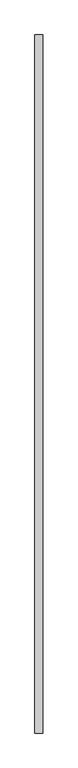
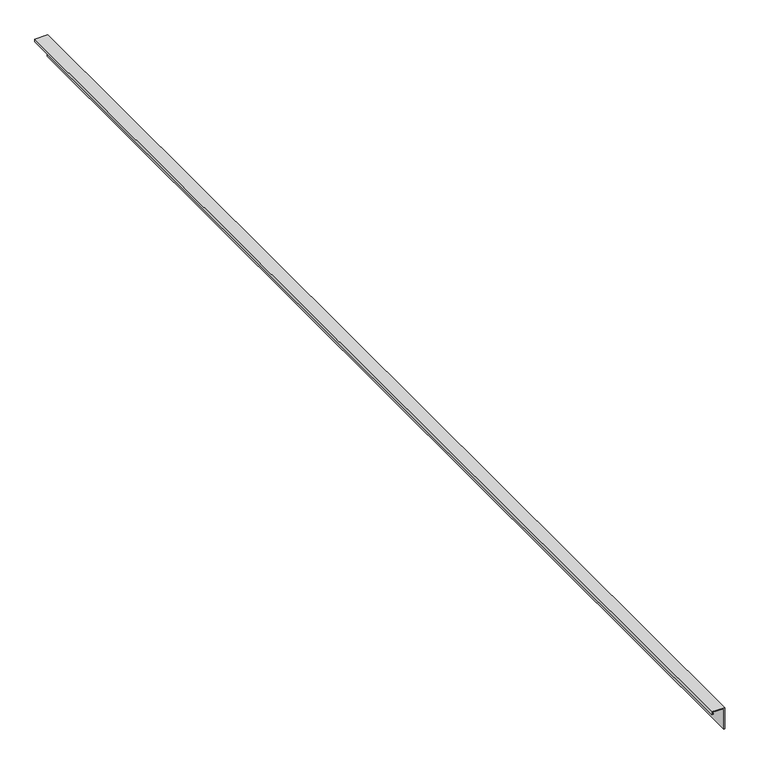
"""IFC4 building model written with IfcOpenShell, lengths in millimetres: proxy geometry, GRAVEL STOP18:GRAVEL STOP002:306725 : GRAVEL STOP18:GRAVEL STOP002:306725."""

from ifc_helpers import new_model, si_unit, frame, origin, place, context, project, spatial, polyline, outline, extrude, source, transform, mapped, element, save


def generic_models_a9169bb3(model_context):
    return source(origin(), model_context, "Body", "SweptSolid", [
        extrude(outline(polyline([(40234.4061757, 1966.5954611), (40234.4061757, 1986.2804611), (40197.5761757, 1986.2804611), (40197.5761757, 1987.5504611), (40235.6761757, 1987.5504611), (40235.6761757, 1965.3254611), (40230.9263757, 1965.3254611), (40230.9263757, 1968.3279174), (40232.1963757, 1968.3279174), (40232.1963757, 1966.5954611), (40234.4061757, 1966.5954611)])), frame((0.0, 1278.3325412, 0.0), z_axis=(0.0, 1.0, 0.0), x_axis=(0.0, 0.0, 1.0)), (0.0, 0.0, 1.0), 2000.25),
    ])


if __name__ == "__main__":
    model = new_model("IFC4")
    model_context = context("Model", 3, world=origin())
    ifc_project = project(units=[si_unit("LENGTHUNIT", "METRE", prefix="MILLI")], contexts=[model_context])
    site = spatial("IfcSite", under=ifc_project)
    building = spatial("IfcBuilding", under=site)
    placement = place(None, origin())
    generic_models_shape = generic_models_a9169bb3(model_context)
    element("IfcBuildingElementProxy", 1, Name="GRAVEL STOP18:GRAVEL STOP002:306725 : GRAVEL STOP18:GRAVEL STOP002:306725", ObjectType="GRAVEL STOP18:GRAVEL STOP002:306725 : GRAVEL STOP18:GRAVEL STOP002:306725", at=placement, inside=building, context=model_context, shape_type="MappedRepresentation", body=[
        mapped(generic_models_shape, transform((0.0, 0.0, 0.0), x_axis=(1.0, 0.0, 0.0), y_axis=(0.0, 1.0, 0.0), z_axis=(0.0, 0.0, 1.0))),
    ])
    save(model, "model.ifc")

# Revit data of these elements
# Type "GRAVEL STOP18:GRAVEL STOP002:306725 : GRAVEL STOP18:GRAVEL STOP002:306725"
#   NameOverride = "GRAVEL STOP18:GRAVEL STOP002:306725"
#   ObjectTypeOverride = "GRAVEL STOP18:GRAVEL STOP002"
#   Reference = "GRAVEL STOP002"
#   Category = "Generic Models"
#   Tag = "306725"
# Element 1 (IfcBuildingElementProxy, "GRAVEL STOP18:GRAVEL STOP002:306725 : GRAVEL STOP18:GRAVEL STOP002:306725")
#   Materials on its faces: "COPPER STUCCO J BEAD"
# Materials
#   "COPPER STUCCO J BEAD": class "Unassigned", colour RGB 251 232 155, transparency 0, Cost = 0
